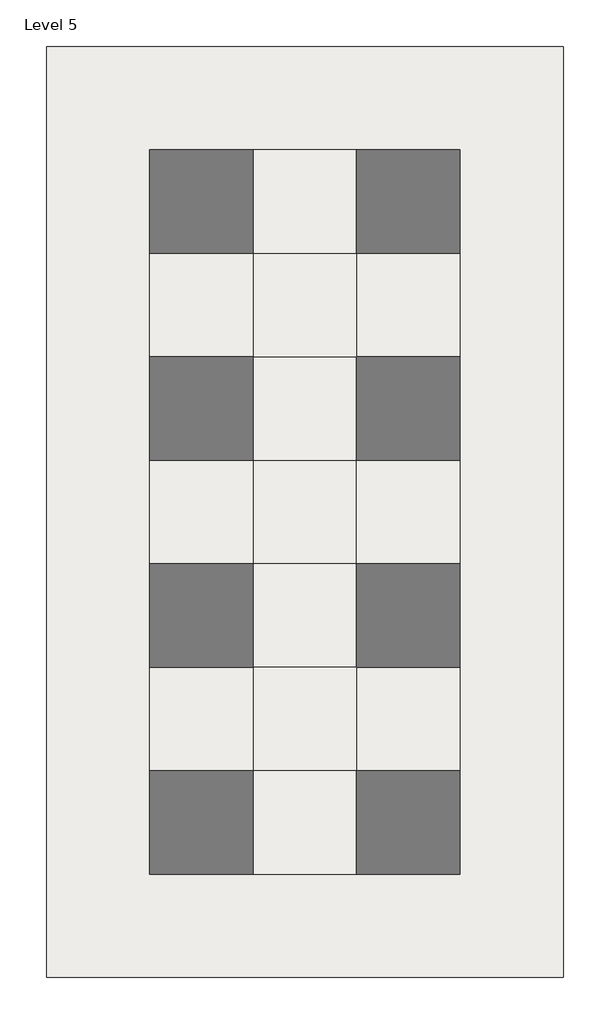
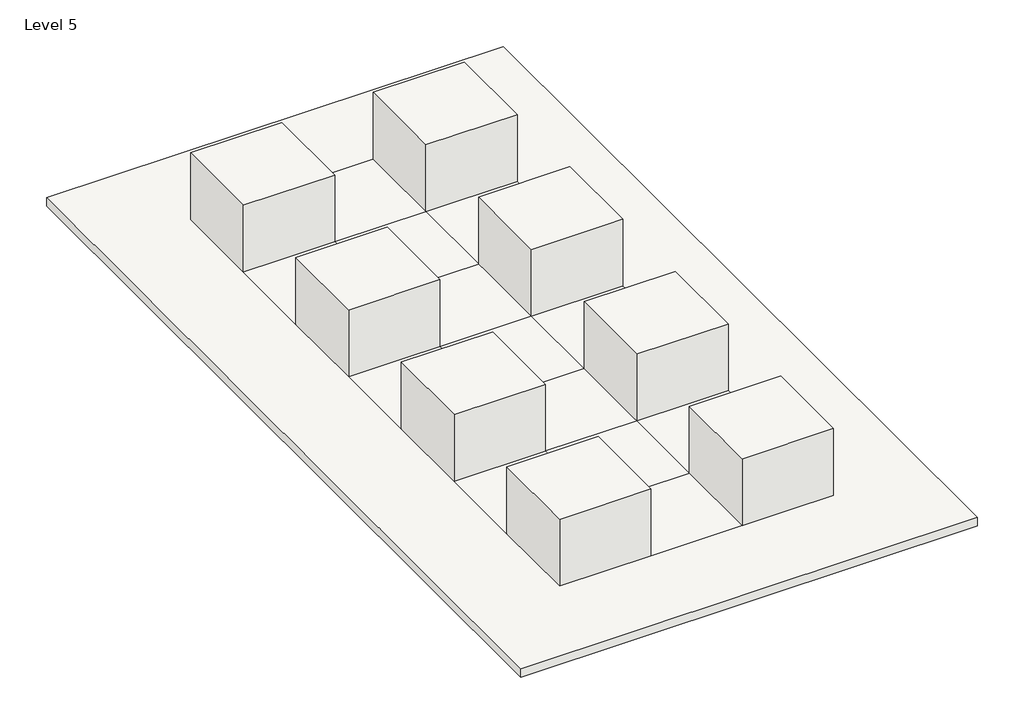
# One storey: 9 roofs.
"""IFC4 building model written with IfcOpenShell, lengths in millimetres."""

from ifc_helpers import new_model, si_unit, origin, place, context, project, spatial, faceted_brep, element, save

model = new_model("IFC4")

# Units and contexts
model_context = context("Model", 3, world=origin())
ifc_project = project(units=[si_unit("LENGTHUNIT", "METRE", prefix="MILLI")], contexts=[model_context])

# Site, building, storey
site = spatial("IfcSite", under=ifc_project)
building = spatial("IfcBuilding", under=site)
storey = spatial("IfcBuildingStorey", under=building, Name="Level 5", Elevation=20000.0)

# Roofs
placement = place(None, origin())
element("IfcRoof", 1, ObjectType="Bauder_RoofCoveringSystem_IntensiveGreenRoofSystem", at=placement, inside=storey, context=model_context, shape_type="Brep", body=[
    faceted_brep([(-674.7340554, 1676.2074539, 20000.0), (1325.2659446, 1676.2074539, 20000.0), (1325.2659446, -323.7925461, 20000.0), (-674.7340554, -323.7925461, 20000.0), (1325.2659446, 1676.2074539, 21749.8), (-674.7340554, 1676.2074539, 21749.8), (-674.7340554, -323.7925461, 21749.8), (1325.2659446, -323.7925461, 21749.8), (1325.2659446, 1676.2074539, 20200.0), (-674.7340554, 1676.2074539, 20200.0), (-674.7340554, -323.7925461, 20200.0), (1325.2659446, -323.7925461, 20200.0)], [[[0, 1, 2, 3]], [[4, 5, 6, 7]], [[5, 4, 8, 1, 0, 9]], [[6, 5, 9, 0, 3, 10]], [[7, 6, 10, 3, 2, 11]], [[4, 7, 11, 2, 1, 8]]]),
])
element("IfcRoof", 2, ObjectType="Bauder_RoofCoveringSystem_IntensiveGreenRoofSystem", at=placement, inside=storey, context=model_context, shape_type="Brep", body=[
    faceted_brep([(3325.2659446, 1676.2074539, 20000.0), (5325.2659446, 1676.2074539, 20000.0), (5325.2659446, -323.7925461, 20000.0), (3325.2659446, -323.7925461, 20000.0), (5325.2659446, 1676.2074539, 21749.8), (3325.2659446, 1676.2074539, 21749.8), (3325.2659446, -323.7925461, 21749.8), (5325.2659446, -323.7925461, 21749.8), (3325.2659446, 1676.2074539, 20200.0), (5325.2659446, 1676.2074539, 20200.0), (3325.2659446, -323.7925461, 20200.0), (5325.2659446, -323.7925461, 20200.0)], [[[0, 1, 2, 3]], [[4, 5, 6, 7]], [[0, 8, 5, 4, 9, 1]], [[3, 10, 6, 5, 8, 0]], [[2, 11, 7, 6, 10, 3]], [[1, 9, 4, 7, 11, 2]]]),
])
element("IfcRoof", 3, ObjectType="Bauder_RoofCoveringSystem_IntensiveGreenRoofSystem", at=placement, inside=storey, context=model_context, shape_type="Brep", body=[
    faceted_brep([(3325.2659446, -2323.7925461, 20000.0), (5325.2659446, -2323.7925461, 20000.0), (5325.2659446, -4323.7925461, 20000.0), (3325.2659446, -4323.7925461, 20000.0), (5325.2659446, -2323.7925461, 21749.8), (3325.2659446, -2323.7925461, 21749.8), (3325.2659446, -4323.7925461, 21749.8), (5325.2659446, -4323.7925461, 21749.8), (3325.2659446, -2323.7925461, 20200.0), (5325.2659446, -2323.7925461, 20200.0), (3325.2659446, -4323.7925461, 20200.0), (5325.2659446, -4323.7925461, 20200.0)], [[[0, 1, 2, 3]], [[4, 5, 6, 7]], [[0, 8, 5, 4, 9, 1]], [[3, 10, 6, 5, 8, 0]], [[2, 11, 7, 6, 10, 3]], [[1, 9, 4, 7, 11, 2]]]),
])
element("IfcRoof", 4, ObjectType="Bauder_RoofCoveringSystem_IntensiveGreenRoofSystem", at=placement, inside=storey, context=model_context, shape_type="Brep", body=[
    faceted_brep([(3325.2659446, -6323.7925461, 20000.0), (5325.2659446, -6323.7925461, 20000.0), (5325.2659446, -8323.7925461, 20000.0), (3325.2659446, -8323.7925461, 20000.0), (5325.2659446, -6323.7925461, 21749.8), (3325.2659446, -6323.7925461, 21749.8), (3325.2659446, -8323.7925461, 21749.8), (5325.2659446, -8323.7925461, 21749.8), (3325.2659446, -6323.7925461, 20200.0), (5325.2659446, -6323.7925461, 20200.0), (3325.2659446, -8323.7925461, 20200.0), (5325.2659446, -8323.7925461, 20200.0)], [[[0, 1, 2, 3]], [[4, 5, 6, 7]], [[0, 8, 5, 4, 9, 1]], [[3, 10, 6, 5, 8, 0]], [[2, 11, 7, 6, 10, 3]], [[1, 9, 4, 7, 11, 2]]]),
])
element("IfcRoof", 5, ObjectType="Bauder_RoofCoveringSystem_IntensiveGreenRoofSystem", at=placement, inside=storey, context=model_context, shape_type="Brep", body=[
    faceted_brep([(3325.2659446, -10323.7925461, 20000.0), (5325.2659446, -10323.7925461, 20000.0), (5325.2659446, -12323.7925461, 20000.0), (3325.2659446, -12323.7925461, 20000.0), (5325.2659446, -10323.7925461, 21749.8), (3325.2659446, -10323.7925461, 21749.8), (3325.2659446, -12323.7925461, 21749.8), (5325.2659446, -12323.7925461, 21749.8), (3325.2659446, -10323.7925461, 20200.0), (5325.2659446, -10323.7925461, 20200.0), (3325.2659446, -12323.7925461, 20200.0), (5325.2659446, -12323.7925461, 20200.0)], [[[0, 1, 2, 3]], [[4, 5, 6, 7]], [[0, 8, 5, 4, 9, 1]], [[3, 10, 6, 5, 8, 0]], [[2, 11, 7, 6, 10, 3]], [[1, 9, 4, 7, 11, 2]]]),
])
element("IfcRoof", 6, ObjectType="Bauder_RoofCoveringSystem_IntensiveGreenRoofSystem", at=placement, inside=storey, context=model_context, shape_type="Brep", body=[
    faceted_brep([(-674.7340554, -10323.7925461, 20000.0), (1325.2659446, -10323.7925461, 20000.0), (1325.2659446, -12323.7925461, 20000.0), (-674.7340554, -12323.7925461, 20000.0), (1325.2659446, -10323.7925461, 21749.8), (-674.7340554, -10323.7925461, 21749.8), (-674.7340554, -12323.7925461, 21749.8), (1325.2659446, -12323.7925461, 21749.8), (-674.7340554, -10323.7925461, 20200.0), (1325.2659446, -10323.7925461, 20200.0), (-674.7340554, -12323.7925461, 20200.0), (1325.2659446, -12323.7925461, 20200.0)], [[[0, 1, 2, 3]], [[4, 5, 6, 7]], [[0, 8, 5, 4, 9, 1]], [[3, 10, 6, 5, 8, 0]], [[2, 11, 7, 6, 10, 3]], [[1, 9, 4, 7, 11, 2]]]),
])
element("IfcRoof", 7, ObjectType="Bauder_RoofCoveringSystem_IntensiveGreenRoofSystem", at=placement, inside=storey, context=model_context, shape_type="Brep", body=[
    faceted_brep([(-674.7340554, -6323.7925461, 20000.0), (1325.2659446, -6323.7925461, 20000.0), (1325.2659446, -8323.7925461, 20000.0), (-674.7340554, -8323.7925461, 20000.0), (1325.2659446, -6323.7925461, 21749.8), (-674.7340554, -6323.7925461, 21749.8), (-674.7340554, -8323.7925461, 21749.8), (1325.2659446, -8323.7925461, 21749.8), (-674.7340554, -6323.7925461, 20200.0), (1325.2659446, -6323.7925461, 20200.0), (-674.7340554, -8323.7925461, 20200.0), (1325.2659446, -8323.7925461, 20200.0)], [[[0, 1, 2, 3]], [[4, 5, 6, 7]], [[0, 8, 5, 4, 9, 1]], [[3, 10, 6, 5, 8, 0]], [[2, 11, 7, 6, 10, 3]], [[1, 9, 4, 7, 11, 2]]]),
])
element("IfcRoof", 8, ObjectType="Bauder_RoofCoveringSystem_IntensiveGreenRoofSystem", at=placement, inside=storey, context=model_context, shape_type="Brep", body=[
    faceted_brep([(-674.7340554, -2323.7925461, 20000.0), (1325.2659446, -2323.7925461, 20000.0), (1325.2659446, -4323.7925461, 20000.0), (-674.7340554, -4323.7925461, 20000.0), (1325.2659446, -2323.7925461, 21749.8), (-674.7340554, -2323.7925461, 21749.8), (-674.7340554, -4323.7925461, 21749.8), (1325.2659446, -4323.7925461, 21749.8), (-674.7340554, -2323.7925461, 20200.0), (1325.2659446, -2323.7925461, 20200.0), (-674.7340554, -4323.7925461, 20200.0), (1325.2659446, -4323.7925461, 20200.0)], [[[0, 1, 2, 3]], [[4, 5, 6, 7]], [[0, 8, 5, 4, 9, 1]], [[3, 10, 6, 5, 8, 0]], [[2, 11, 7, 6, 10, 3]], [[1, 9, 4, 7, 11, 2]]]),
])
element("IfcRoof", 9, ObjectType="Roof_Concrete-200mm", at=placement, inside=storey, context=model_context, shape_type="Brep", body=[
    faceted_brep([(-2674.7340554, -14323.7925461, 20200.0), (-2674.7340554, -14323.7925461, 20000.0), (7325.2659446, -14323.7925461, 20000.0), (7325.2659446, -14323.7925461, 20200.0), (-2674.7340554, 3676.2074539, 20200.0), (-2674.7340554, 3676.2074539, 20000.0), (7325.2659446, 3676.2074539, 20200.0), (7325.2659446, 3676.2074539, 20000.0), (3325.2659446, 1676.2074539, 20200.0), (1325.2659446, 1676.2074539, 20200.0), (1325.2659446, -323.7925461, 20200.0), (3325.2659446, -323.7925461, 20200.0), (1325.2659446, 1676.2074539, 20000.0), (3325.2659446, 1676.2074539, 20000.0), (3325.2659446, -323.7925461, 20000.0), (1325.2659446, -323.7925461, 20000.0), (1325.2659446, -2323.7925461, 20200.0), (-674.7340554, -323.7925461, 20200.0), (-674.7340554, -2323.7925461, 20200.0), (3325.2659446, -2323.7925461, 20200.0), (5325.2659446, -2323.7925461, 20200.0), (5325.2659446, -323.7925461, 20200.0), (-674.7340554, -2323.7925461, 20000.0), (-674.7340554, -323.7925461, 20000.0), (1325.2659446, -2323.7925461, 20000.0), (3325.2659446, -2323.7925461, 20000.0), (5325.2659446, -323.7925461, 20000.0), (5325.2659446, -2323.7925461, 20000.0), (1325.2659446, -4323.7925461, 20200.0), (3325.2659446, -4323.7925461, 20200.0), (3325.2659446, -4323.7925461, 20000.0), (1325.2659446, -4323.7925461, 20000.0), (1325.2659446, -6323.7925461, 20200.0), (-674.7340554, -4323.7925461, 20200.0), (-674.7340554, -6323.7925461, 20200.0), (5325.2659446, -6323.7925461, 20200.0), (5325.2659446, -4323.7925461, 20200.0), (3325.2659446, -6323.7925461, 20200.0), (-674.7340554, -6323.7925461, 20000.0), (-674.7340554, -4323.7925461, 20000.0), (1325.2659446, -6323.7925461, 20000.0), (3325.2659446, -6323.7925461, 20000.0), (5325.2659446, -4323.7925461, 20000.0), (5325.2659446, -6323.7925461, 20000.0), (1325.2659446, -12323.7925461, 20200.0), (3325.2659446, -12323.7925461, 20200.0), (3325.2659446, -10323.7925461, 20200.0), (1325.2659446, -10323.7925461, 20200.0), (3325.2659446, -12323.7925461, 20000.0), (1325.2659446, -12323.7925461, 20000.0), (1325.2659446, -10323.7925461, 20000.0), (3325.2659446, -10323.7925461, 20000.0), (1325.2659446, -8323.7925461, 20200.0), (-674.7340554, -8323.7925461, 20200.0), (-674.7340554, -10323.7925461, 20200.0), (3325.2659446, -8323.7925461, 20200.0), (5325.2659446, -10323.7925461, 20200.0), (5325.2659446, -8323.7925461, 20200.0), (-674.7340554, -10323.7925461, 20000.0), (-674.7340554, -8323.7925461, 20000.0), (1325.2659446, -8323.7925461, 20000.0), (3325.2659446, -8323.7925461, 20000.0), (5325.2659446, -8323.7925461, 20000.0), (5325.2659446, -10323.7925461, 20000.0), (-674.7340554, 1676.2074539, 20000.0), (-674.7340554, 1676.2074539, 20200.0), (5325.2659446, 1676.2074539, 20200.0), (5325.2659446, 1676.2074539, 20000.0), (5325.2659446, -12323.7925461, 20000.0), (5325.2659446, -12323.7925461, 20200.0), (-674.7340554, -12323.7925461, 20000.0), (-674.7340554, -12323.7925461, 20200.0)], [[[0, 1, 2, 3]], [[1, 0, 4, 5]], [[6, 7, 5, 4]], [[3, 2, 7, 6]], [[8, 9, 10, 11]], [[12, 13, 14, 15]], [[16, 10, 17, 18]], [[11, 10, 16, 19]], [[20, 21, 11, 19]], [[22, 23, 15, 24]], [[15, 14, 25, 24]], [[25, 14, 26, 27]], [[19, 16, 28, 29]], [[24, 25, 30, 31]], [[32, 28, 33, 34]], [[35, 36, 29, 37]], [[38, 39, 31, 40]], [[41, 30, 42, 43]], [[44, 45, 46, 47]], [[48, 49, 50, 51]], [[47, 52, 53, 54]], [[47, 46, 55, 52]], [[56, 57, 55, 46]], [[58, 59, 60, 50]], [[51, 50, 60, 61]], [[51, 61, 62, 63]], [[52, 55, 37, 32]], [[29, 28, 32, 37]], [[61, 60, 40, 41]], [[31, 30, 41, 40]], [[9, 12, 15, 10]], [[10, 15, 23, 17]], [[17, 23, 64, 65]], [[12, 9, 65, 64]], [[66, 67, 26, 21]], [[21, 26, 14, 11]], [[11, 14, 13, 8]], [[67, 66, 8, 13]], [[20, 27, 42, 36]], [[36, 42, 30, 29]], [[29, 30, 25, 19]], [[27, 20, 19, 25]], [[16, 24, 31, 28]], [[28, 31, 39, 33]], [[33, 39, 22, 18]], [[24, 16, 18, 22]], [[32, 40, 60, 52]], [[52, 60, 59, 53]], [[53, 59, 38, 34]], [[40, 32, 34, 38]], [[35, 43, 62, 57]], [[57, 62, 61, 55]], [[55, 61, 41, 37]], [[43, 35, 37, 41]], [[56, 63, 68, 69]], [[69, 68, 48, 45]], [[45, 48, 51, 46]], [[63, 56, 46, 51]], [[47, 50, 49, 44]], [[44, 49, 70, 71]], [[71, 70, 58, 54]], [[50, 47, 54, 58]], [[4, 0, 3, 6], [9, 8, 66, 21, 20, 36, 35, 57, 56, 69, 45, 44, 71, 54, 53, 34, 33, 18, 17, 65]], [[7, 2, 1, 5], [13, 12, 64, 23, 22, 39, 38, 59, 58, 70, 49, 48, 68, 63, 62, 43, 42, 27, 26, 67]]]),
])

save(model, "model.ifc")

# Revit data of these elements
# Type "Bauder_RoofCoveringSystem_IntensiveGreenRoofSystem"
#   Keynote = "Q37"
#   Type IFC Predefined Type = "FLAT_ROOF"
#   Export Type to IFC As = "IfcRoofType"
#   Model = "Bauder Intensive Landscaping and Substrate - Intensive Green Roof System"
#   Manufacturer = "Bauder Ltd"
#   Type Comments = "Intensive Green Roof System"
#   URL = "http://www.bauder.co.uk/"
#   Description = "Bauder Intensive GreenRoof system incorporating Intensive Landscaping with Intensive Substrate, Filter Fleece, Mineral Drain, DSE60 Polyethylene Drainage and Protection Layer, FSM 1100 protection mat and PE Foil Polyethylene Separation-Slip Layer"
#   Assembly Code = "B3010"
#   NBSDescription = "Intensive green roof system"
#   NBSReference = "45-40-47/110"
#   BIMObjectName = "Bauder_RoofCoveringSystem_IntensiveGreenRoofSystem"
#   AccessibilityPerformance = "n/a"
#   CodePerformance = "n/a"
#   Color = "n/a"
#   Constituents = "n/a"
#   DurationUnit = "Year"
#   ExpectedLife = "n/a"
#   Features = "This BIM Object must be supported by a project specific specification from Bauder, incorporating system build-up, detail design and performance calculations if a full Bauder system guarantee is required. Please contact your local Bauder Representative or technical@bauder.co.uk"
#   Finish = "n/a"
#   Grade = "n/a"
#   Material = "n/a"
#   ModelReference = "Bauder Intensive Landscaping and Substrate - Intensive Green Roof System"
#   Name = "RoofCoveringSystem_Bauder_IntensiveGreenRoofSystem"
#   ReplacementCost = "n/a"
#   Shape = "n/a"
#   Size = "n/a"
#   SustainabilityPerformance = "Bauder Germany ISO14001: Certificate No.: 70499/03-15 e, Bauder UK ISO14001:Certificate No. 19ACM6595R, EN1271, BREEAM Credits Available"
#   WarrantyDescription = "Guarantee options could include ‘Product’, ‘Product and Workmanship’ and ‘Product, Workmanship and Design’ Guarantees. All guarantees available for this system are subject to the works being carried out in accordance with the Bauder specification and being installed by a Bauder Approved installer. For full details and further information regarding guarantees and alternative systems please contact your local Bauder Representative or technical@bauder.co.uk"
#   WarrantyDurationLabor = "n/a"
#   WarrantyDurationParts = "n/a\r\nn/a"
#   WarrantyDurationUnit = "Year"
#   WarrantyGuarantorLabor = "n/a"
#   WarrantyGuarantorParts = "technical@bauder.co.uk"
#   Certification = "n/a"
#   EdgeRestraints = "Perforated edge trim where required, refer to Bauder Project Specific Specification"
#   MoistureControlDrainageAncillaries = "n/a"
#   MoistureControlDrainageLayer = "Bauder DSE60 60 mm Polyethylene Drainage and Protection Layer with Bauder Mineral Drain Single size stone aggregate infill"
#   MoistureControlFilterMembrane = "Bauder Filter Fleece 1 mm Polypropylene Filter Fleece"
#   MoistureControlMoistureRetentionMat = "n/a"
#   PlantingSystemsAntierosionMat = "Jute Net where exposed, refer to Bauder Project Specific Specification"
#   PlantingSystemsPlantingMedium = "Bauder Intensive Substrate Recycled crushed brick, expanded clay shale and composted pine bark"
#   PlantingSystemsVegetation = "Bauder Intensive Landscaping"
#   PlantingSystemsVegetationBarrier = "20-40 mm Rounded-Washed Stones, refer to Bauder Project Specific Specification"
#   ProjectSpecificationAndDesign = "This BIM Object must be supported by a project specific specification from Bauder, incorporating system build-up, detail design and performance calculations if a full Bauder system warranty is required. Please contact your local Bauder Representative or technical@bauder.co.uk"
#   ProtectionProtectionLayer = "BauderGREEN FSM 1100 Protection Mat"
#   ProtectionRootBarrier = "As per project specific Bauder Specification"
#   ProtectionSeparationLayer = "2 layers of Bauder PE Foil 0.2 mm Polyethylene Separation-Slip Layer"
#   SystemManufacturer = "Bauder Ltd"
#   WarrantyConsiderations = "All guarantees available for this system are subject to the works being carried out in accordance with the Bauder specification and being installed by a Bauder Approved installer. For full details and further information regarding guarantees and alternative systems please contact your local Bauder Representative or technical@bauder.co.uk"
#   Update = "1900-12-31T23:59:59"
#   Documentation = "https://www.bauder.co.uk/technical-centre/technical-literature/system-brochures"
#   DocumentReference = "http://www.bauder.co.uk/"
#   IfcExportAs = "IfcRoofType"
#   IfcExportType = "FLAT_ROOF"
#   MethodOfMesurement = "n/a"
#   Process = "Replacement at service life intervals"
#   FireRating = "n/a"
#   _Author = "AM"
#   _AuthorizedBy = "bimstore"
#   _CreatedBy = "technical@bauder.co.uk"
#   _DistributedBy = "www.bimstore.co"
#   AssetType = "Fixed"
#   ClassificationName = "Uniclass2015"
#   ClassificationValue = "Ss_45_40_47_40"
#   CreatedBy = "technical@bauder.co.uk"
#   CreatedOn = "2023-02-10 T00:00:00"
#   DocumentationCertificates = "n/a"
#   DocumentationInstallationGuide = "https://www.bauder.co.uk/technical-centre"
#   DocumentationLiterature = "https://www.bauder.co.uk/technical-centre"
#   DocumentationMaintenance = "https://www.bauder.co.uk/technical-centre/maintenance-advice"
#   DocumentationTechnical = "https://www.bauder.co.uk/green-roofs/intensive-green-roofs"
#   ManufacturerName = "Bauder Ltd"
#   ModelNumber = "0910_INT-InS-FF-D6-F11-PE"
#   ProductionYear = "2023"
#   ReferencedStandard = "n/a"
#   SpareParts = "n/a"
#   TypeName = "Intensive Green Roof System"
#   NBSNote = "n/a"
#   NBSObjectName = "Bauder - Intensive green roof system"
#   NBSOfficeMasterTag = "n/a"
#   Ballast = "n/a"
#   CarrierMembraneFixing = "n/a"
#   CarrierMembraneType = "n/a"
#   FillToPerimeterUpstands = "n/a"
#   FilterLayer = "n/a"
#   InsulationFixing = "n/a"
#   InsulationType = "n/a"
#   LiquidAppliedWaterproofCoatingReinforcement = "n/a"
#   LiquidAppliedWaterproofCoatingSurfaceTreatment = "n/a"
#   LiquidAppliedWaterproofCoatingType = "n/a"
#   PreparationExistingSubstrates = "n/a"
#   PreparationHorizontalWork = "n/a"
#   PreparationSkirtingsAndVerticalWork = "n/a"
#   ProtectionLayer = "n/a"
#   SystemAccessories = "n/a"
#   WaterproofCoveringFirstLayerAttachment = "n/a"
#   WaterproofCoveringFirstLayerType = "n/a"
#   WaterproofCoveringIntermediateLayerAttachment = "n/a"
#   WaterproofCoveringIntermediateLayerType = "n/a"
#   WaterproofCoveringTopLayerAttachment = "n/a"
#   InsulationAttachment = "n/a"
#   IsolatingLayer = "n/a"
#   CarrierMembraneAttachment = "n/a"
#   LiquidAppliedWaterproofCoatingWearingCourse = "n/a"
#   VapourControlLayer = "n/a"
#   VapourControlLayerAttachment_Bauder = "n/a"
#   WaterproofCoveringJoints = "n/a"
#   WaterproofCoveringType = "n/a"
#   SeparatingLayer = "n/a"
#   WaterproofCoveringAccessories = "Yes"
#   WaterproofCoveringAttachment = "n/a"
#   UpperProtectionLayer = "n/a"
#   LowerProtectionLayer = "n/a"
#   WaterproofCoveringTopLayerType = "n/a"
#   DetailWorkAncillaryItems = "Detail as per project specific Bauder Specification"
#   DetailWorkCoverStrips = "Detail as per project specific Bauder Specification"
#   DetailWorkFlashings = "Detail as per project specific Bauder Specification"
#   DetailWorkSkirtingsAndUpstands = "Detail as per project specific Bauder Specification"
#   DetailWorkWeltedDrips = "Detail as per project specific Bauder Specification"
#   OverlayFixing = "n/a"
#   OverlayType = "n/a"
#   SurfaceProtection = "n/a"
#   VapourControlLayerAttachment = "n/a"
#   VapourControlLayerType = "n/a"
#   Cost = 0
#   NominalHeight = 0 mm
#   NominalLength = 0 mm
#   TotalArea = 0 m²
#   NominalDepth = 0 mm
#   IsExternal = yes
#   _BimSpecGuid = 0
#   _BSBibleVersion = 16
#   _CurrentRevision = 4
#   Layers, outside or top first: 700 mm "Bauder_Landscaping_Intensive" (function 5); 800 mm "Bauder_IntensiveSubstrate_BauderGREEN-SUB-IM-UK" (function 2); 1 mm "Bauder_FilterFleece_BauderGREEN-FV-125-100" (function 2); 40 mm "Bauder_DrainageBoard_BauderGREEN-DSE-40" (function 3); 8 mm "Bauder_ProtectionMat_BauderGREEN-FSM1100" (function 3); 200 mm "Concrete" (function 1); 0.8 mm "Bauder_SeparationAndSlipLayer_BauderGREEN-PE-02" (function 3)
# Type "Roof_Concrete-200mm"
#   Layers, outside or top first: 200 mm "Concrete" (function 1)
# Elements 1, 2, 3, 4, 5, 6, 7, 8 (IfcRoof, "Bauder_RoofCoveringSystem_IntensiveGreenRoofSystem")
#   built-in parameter 1001705 = 71.3576 (stored number, unit not read)
#   built-in parameter 1001710 = 33615
#   Phase Created = New Construction
#   Materials on its faces: "Bauder_SeparationAndSlipLayer_BauderGREEN-PE-02", "Bauder_Landscaping_Intensive"
# Element 9 (IfcRoof, "Roof_Concrete-200mm")
#   built-in parameter 1001710 = 33615
#   Phase Created = New Construction
#   Materials on its faces: "Concrete"
# Materials
#   "Bauder_Landscaping_Intensive": class "Unassigned", colour RGB 62 68 37, transparency 0, Mtrl_Author = "AM", Mtrl_AuthorizedBy = "bimstore", Mtrl_DistributedBy = "www.bimstore.co", Mtrl_AccessibilityPerformance = "n/a", Mtrl_AssetIdentifier = "Please record on commissioning", Mtrl_AssetType = "Fixed", Mtrl_BarCode = "Please record on commissioning", Mtrl_ClassificationName = "Uniclass2015", Mtrl_ClassificationValue = "n/a", Mtrl_CodePerformance = "n/a", Mtrl_Color = "n/a", Mtrl_Constituents = "n/a", Mtrl_CreatedBy = "technical@bauder.co.uk", Mtrl_CreatedOn = "2023-02-10 T00:00:00", Mtrl_DocumentationCertificates = "https://www.bimstore.co/products/intensive-green-roof-system/document/product-certificates", Mtrl_DocumentationInstallationGuide = "https://www.bimstore.co/products/intensive-green-roof-system/document/installation-guide", Mtrl_DocumentationLiterature = "https://www.bimstore.co/products/intensive-green-roof-system/document/product-literature", Mtrl_DocumentationMaintenance = "https://www.bimstore.co/products/intensive-green-roof-system/document/maintenance-information", Mtrl_DocumentationTechnical = "https://www.bimstore.co/products/intensive-green-roof-system/document/technical-data-sheet", Mtrl_DurationUnit = "Year", Mtrl_Features = "n/a", Mtrl_Finish = "n/a", Mtrl_Grade = "n/a", Mtrl_InstallationDate = "Please record on commissioning", Mtrl_ManufacturerName = "Bauder Ltd", Mtrl_Material = "n/a", Mtrl_ModelNumber = "Intensive", Mtrl_ModelReference = "Landscaping", Mtrl_ProductionYear = "2023", Mtrl_ReferencedStandard = "n/a", Mtrl_Shape = "n/a", Mtrl_Size = "n/a", Mtrl_SpareParts = "n/a", Mtrl_TypeName = "Intensive", Mtrl_WarrantyDescription = "n/a", Mtrl_WarrantyDurationUnit = "Year", Mtrl_WarrantyGuarantorLabor = "n/a", Mtrl_WarrantyGuarantorParts = "technical@bauder.co.uk", Mtrl_WarrantyStartDate = "Please record on commissioning", Mtrl_IfcExportAs = "IfcRoofType", Mtrl_IfcExportType = "FLAT_ROOF", Mtrl_BIMObjectName = "Bauder_Landscaping_Intensive", Mtrl_NBSDescription = "n/a", Mtrl_NBSNote = "n/a", Mtrl_NBSObjectName = "n/a", Mtrl_NBSOfficeMasterTag = "n/a", Mtrl_NBSReference = "Q37", Mtrl_Ballast = "n/a", Mtrl_CarrierMembraneAttachment = "n/a", Mtrl_CarrierMembraneFixing = "n/a", Mtrl_CarrierMembraneType = "n/a", Mtrl_Certification = "Comply with GRO Green Roof Code of Practice and FLL Standards", Mtrl_DetailWorkAncillaryItems = "Detail as per project specific Bauder Specification", Mtrl_DetailWorkCoverStrips = "Detail as per project specific Bauder Specification", Mtrl_DetailWorkFlashings = "Detail as per project specific Bauder Specification", Mtrl_DetailWorkSkirtingsAndUpstands = "Detail as per project specific Bauder Specification", Mtrl_DetailWorkWeltedDrips = "Detail as per project specific Bauder Specification", Mtrl_EdgeRestraints = "Detail as per project specific Bauder Specification", Mtrl_FillToPerimeterUpstands = "n/a", Mtrl_FilterLayer = "n/a", Mtrl_InsulationAttachment = "As per project specific Bauder Specification", Mtrl_InsulationFixing = "As per project specific Bauder Specification", Mtrl_InsulationType = "As per project specific Bauder Specification", Mtrl_IsolatingLayer = "n/a", Mtrl_LiquidAppliedWaterproofCoatingReinforcement = "n/a", Mtrl_LiquidAppliedWaterproofCoatingSurfaceTreatment = "As per project specific Bauder Specification", Mtrl_LiquidAppliedWaterproofCoatingType = "As per project specific Bauder Specification", Mtrl_LiquidAppliedWaterproofCoatingWearingCourse = "As per project specific Bauder Specification", Mtrl_LowerProtectionLayer = "n/a", Mtrl_MoistureControlDrainageAncillaries = "n/a", Mtrl_MoistureControlDrainageLayer = "n/a", Mtrl_MoistureControlFilterMembrane = "n/a", Mtrl_MoistureControlMoistureRetentionMat = "n/a", Mtrl_OverlayFixing = "n/a", Mtrl_OverlayType = "n/a", Mtrl_PlantingSystemsAntierosionMat = "n/a", Mtrl_PlantingSystemsPlantingMedium = "As per project specific Bauder Specification", Mtrl_PlantingSystemsVegetation = "As per project specific Bauder Specification", Mtrl_PlantingSystemsVegetationBarrier = "As per project specific Bauder Specification", Mtrl_PreparationExistingSubstrates = "n/a", Mtrl_PreparationHorizontalWork = "n/a", Mtrl_PreparationSkirtingsAndVerticalWork = "n/a", Mtrl_ProjectSpecificationAndDesign = "This BIM Object must be supported by a project specific specification from Bauder, incorporating system build-up, detail design and performance calculations if a full Bauder system warranty is required. Please contact your local Bauder Representative or technical@bauder.co.uk", Mtrl_ProtectionLayer = "n/a", Mtrl_ProtectionProtectionLayer = "n/a", Mtrl_ProtectionRootBarrier = "As per project specific Bauder Specification", Mtrl_ProtectionSeparationLayer = "n/a", Mtrl_SeparatingLayer = "n/a", Mtrl_SurfaceProtection = "n/a", Mtrl_SystemAccessories = "n/a", Mtrl_SystemManufacturer = "Bauder Ltd", Mtrl_Update = "1900-12-31 T23:59:59", Mtrl_UpperProtectionLayer = "n/a", Mtrl_VapourControlLayerAttachment = "As per project specific Bauder Specification", Mtrl_VapourControlLayerAttachment_Bauder = "As per project specific Bauder Specification", Mtrl_VapourControlLayerType = "As per project specific Bauder Specification", Mtrl_WarrantyConsiderations = "All guarantees available for this system are subject to the works being carried out in accordance with the Bauder specification and being installed by a Bauder Approved installer. For full details and further information regarding guarantees and alternative systems please contact your local Bauder Representative or technical@bauder.co.uk", Mtrl_WaterproofCoveringAccessories = "As per project specific Bauder Specification", Mtrl_WaterproofCoveringAttachment = "As per project specific Bauder Specification", Mtrl_WaterproofCoveringFirstLayerAttachment = "As per project specific Bauder Specification", Mtrl_WaterproofCoveringFirstLayerType = "As per project specific Bauder Specification", Mtrl_WaterproofCoveringIntermediateLayerAttachment = "As per project specific Bauder Specification", Mtrl_WaterproofCoveringIntermediateLayerType = "As per project specific Bauder Specification", Mtrl_WaterproofCoveringJoints = "As per project specific Bauder Specification", Mtrl_WaterproofCoveringTopLayerAttachment = "As per project specific Bauder Specification", Mtrl_WaterproofCoveringTopLayerType = "As per project specific Bauder Specification", Mtrl_WaterproofCoveringType = "As per project specific Bauder Specification", Cost = 0, Mtrl_ReplacementCost = 0, Mtrl_NominalDepth = 0 mm, Mtrl_NominalHeight = 0 mm, Mtrl_NominalLength = 0 mm, Mtrl_BimSpecGuid = 0, Mtrl_BSBibleVersion = 17, Mtrl_CurrentRevision = 2, Mtrl_ExpectedLife = 0, Mtrl_SerialNumber = 0, Mtrl_WarrantyDurationLabor = 0, Mtrl_WarrantyDurationParts = 0
#   "Bauder_IntensiveSubstrate_BauderGREEN-SUB-IM-UK": class "Unassigned", colour RGB 255 255 255, transparency 0, Mtrl_Author = "AM", Mtrl_AuthorizedBy = "bimstore", Mtrl_DistributedBy = "www.bimstore.co", Mtrl_AccessibilityPerformance = "n/a", Mtrl_AssetIdentifier = "Please record on commissioning", Mtrl_AssetType = "Fixed", Mtrl_BarCode = "Please record on commissioning", Mtrl_ClassificationName = "Uniclass2015", Mtrl_ClassificationValue = "n/a", Mtrl_CodePerformance = "n/a", Mtrl_Color = "n/a", Mtrl_Constituents = "n/a", Mtrl_CreatedBy = "technical@bauder.co.uk", Mtrl_CreatedOn = "2023-02-10 T00:00:00", Mtrl_DocumentationCertificates = "https://www.bimstore.co/products/intensive-green-roof-system/document/product-certificates", Mtrl_DocumentationInstallationGuide = "https://www.bimstore.co/products/intensive-green-roof-system/document/installation-guide", Mtrl_DocumentationLiterature = "https://www.bimstore.co/products/intensive-green-roof-system/document/product-literature", Mtrl_DocumentationMaintenance = "https://www.bimstore.co/products/intensive-green-roof-system/document/maintenance-information", Mtrl_DocumentationTechnical = "https://www.bimstore.co/products/intensive-green-roof-system/document/technical-data-sheet", Mtrl_DurationUnit = "Year", Mtrl_Features = "n/a", Mtrl_Finish = "n/a", Mtrl_Grade = "n/a", Mtrl_InstallationDate = "Please record on commissioning", Mtrl_ManufacturerName = "Bauder Ltd", Mtrl_Material = "Expanded Clay Aggregate", Mtrl_ModelNumber = "BauderGREEN-SUB-IM-UK", Mtrl_ModelReference = "Intensive Substrate", Mtrl_ProductionYear = "2023", Mtrl_ReferencedStandard = "n/a", Mtrl_Shape = "n/a", Mtrl_Size = "n/a", Mtrl_SpareParts = "n/a", Mtrl_TypeName = "BauderGREEN-SUB-IM-UK", Mtrl_WarrantyDescription = "As part of Bauder system guarantee, per specification", Mtrl_WarrantyDurationUnit = "Year", Mtrl_WarrantyGuarantorLabor = "n/a", Mtrl_WarrantyGuarantorParts = "technical@bauder.co.uk", Mtrl_WarrantyStartDate = "Please record on commissioning", Mtrl_IfcExportAs = "IfcRoofType", Mtrl_IfcExportType = "FLAT_ROOF", Mtrl_BIMObjectName = "Bauder_IntensiveSubstrate_BauderGREEN-SUB-IM-UK", Mtrl_NBSDescription = "n/a", Mtrl_NBSNote = "n/a", Mtrl_NBSObjectName = "n/a", Mtrl_NBSOfficeMasterTag = "n/a", Mtrl_NBSReference = "Q37", Mtrl_Ballast = "n/a", Mtrl_CarrierMembraneAttachment = "n/a", Mtrl_CarrierMembraneFixing = "n/a", Mtrl_CarrierMembraneType = "n/a", Mtrl_Certification = "Comply with GRO Green Roof Code of Practice and FLL Standards", Mtrl_DetailWorkAncillaryItems = "Detail as per project specific Bauder Specification", Mtrl_DetailWorkCoverStrips = "Detail as per project specific Bauder Specification", Mtrl_DetailWorkFlashings = "Detail as per project specific Bauder Specification", Mtrl_DetailWorkSkirtingsAndUpstands = "Detail as per project specific Bauder Specification", Mtrl_DetailWorkWeltedDrips = "Detail as per project specific Bauder Specification", Mtrl_EdgeRestraints = "Detail as per project specific Bauder Specification", Mtrl_FillToPerimeterUpstands = "n/a", Mtrl_FilterLayer = "n/a", Mtrl_InsulationAttachment = "As per project specific Bauder Specification", Mtrl_InsulationFixing = "As per project specific Bauder Specification", Mtrl_InsulationType = "As per project specific Bauder Specification", Mtrl_IsolatingLayer = "n/a", Mtrl_LiquidAppliedWaterproofCoatingReinforcement = "As per project specific Bauder Specification", Mtrl_LiquidAppliedWaterproofCoatingSurfaceTreatment = "As per project specific Bauder Specification", Mtrl_LiquidAppliedWaterproofCoatingType = "As per project specific Bauder Specification", Mtrl_LiquidAppliedWaterproofCoatingWearingCourse = "As per project specific Bauder Specification", Mtrl_LowerProtectionLayer = "n/a", Mtrl_MoistureControlDrainageAncillaries = "n/a", Mtrl_MoistureControlDrainageLayer = "n/a", Mtrl_MoistureControlFilterMembrane = "n/a", Mtrl_MoistureControlMoistureRetentionMat = "n/a", Mtrl_OverlayFixing = "n/a", Mtrl_OverlayType = "n/a", Mtrl_PlantingSystemsAntierosionMat = "n/a", Mtrl_PlantingSystemsPlantingMedium = "As per project specific Bauder Specification", Mtrl_PlantingSystemsVegetation = "As per project specific Bauder Specification", Mtrl_PlantingSystemsVegetationBarrier = "As per project specific Bauder Specification", Mtrl_PreparationExistingSubstrates = "n/a", Mtrl_PreparationHorizontalWork = "n/a", Mtrl_PreparationSkirtingsAndVerticalWork = "n/a", Mtrl_ProjectSpecificationAndDesign = "This BIM Object must be supported by a project specific specification from Bauder, incorporating system build-up, detail design and performance calculations if a full Bauder system warranty is required. Please contact your local Bauder Representative or technical@bauder.co.uk", Mtrl_ProtectionLayer = "n/a", Mtrl_ProtectionProtectionLayer = "n/a", Mtrl_ProtectionRootBarrier = "As per project specific Bauder Specification", Mtrl_ProtectionSeparationLayer = "n/a", Mtrl_SeparatingLayer = "n/a", Mtrl_SurfaceProtection = "n/a", Mtrl_SystemAccessories = "n/a", Mtrl_SystemManufacturer = "Bauder Ltd", Mtrl_Update = "1900-12-31 T23:59:59", Mtrl_UpperProtectionLayer = "n/a", Mtrl_VapourControlLayerAttachment = "As per project specific Bauder Specification", Mtrl_VapourControlLayerAttachment_Bauder = "As per project specific Bauder Specification", Mtrl_VapourControlLayerType = "As per project specific Bauder Specification", Mtrl_WarrantyConsiderations = "All guarantees available for this system are subject to the works being carried out in accordance with the Bauder specification and being installed by a Bauder Approved installer. For full details and further information regarding guarantees and alternative systems please contact your local Bauder Representative or technical@bauder.co.uk", Mtrl_WaterproofCoveringAccessories = "As per project specific Bauder Specification", Mtrl_WaterproofCoveringAttachment = "As per project specific Bauder Specification", Mtrl_WaterproofCoveringFirstLayerAttachment = "As per project specific Bauder Specification", Mtrl_WaterproofCoveringFirstLayerType = "As per project specific Bauder Specification", Mtrl_WaterproofCoveringIntermediateLayerAttachment = "As per project specific Bauder Specification", Mtrl_WaterproofCoveringIntermediateLayerType = "As per project specific Bauder Specification", Mtrl_WaterproofCoveringJoints = "As per project specific Bauder Specification", Mtrl_WaterproofCoveringTopLayerAttachment = "As per project specific Bauder Specification", Mtrl_WaterproofCoveringTopLayerType = "As per project specific Bauder Specification", Mtrl_WaterproofCoveringType = "As per project specific Bauder Specification", Cost = 0, Mtrl_ReplacementCost = 0, Mtrl_NominalDepth = 200 mm, Mtrl_NominalHeight = 0 mm, Mtrl_NominalLength = 0 mm, Mtrl_BimSpecGuid = 0, Mtrl_BSBibleVersion = 17, Mtrl_CurrentRevision = 2, Mtrl_ExpectedLife = 0, Mtrl_SerialNumber = 0, Mtrl_WarrantyDurationLabor = 0, Mtrl_WarrantyDurationParts = 0
#   "Bauder_FilterFleece_BauderGREEN-FV-125-100": class "Unassigned", colour RGB 255 255 255, transparency 0, Mtrl_Author = "AM", Mtrl_AuthorizedBy = "bimstore", Mtrl_DistributedBy = "www.bimstore.co", Mtrl_AccessibilityPerformance = "n/a", Mtrl_AssetIdentifier = "Please record on commissioning", Mtrl_AssetType = "Fixed", Mtrl_BarCode = "Please record on commissioning", Mtrl_ClassificationName = "Uniclass2015", Mtrl_ClassificationValue = "n/a", Mtrl_CodePerformance = "n/a", Mtrl_Color = "n/a", Mtrl_Constituents = "n/a", Mtrl_CreatedBy = "technical@bauder.co.uk", Mtrl_CreatedOn = "2023-02-10 T00:00:00", Mtrl_DocumentationCertificates = "https://www.bimstore.co/products/extensive-green-roof-system-wildflower-blanket/document/product-certificates", Mtrl_DocumentationInstallationGuide = "https://www.bimstore.co/products/extensive-green-roof-system-wildflower-blanket/document/installation-guide", Mtrl_DocumentationLiterature = "https://www.bimstore.co/products/intensive-green-roof-system/document/product-literature", Mtrl_DocumentationMaintenance = "https://www.bimstore.co/products/extensive-green-roof-system-wildflower-blanket/document/maintenance-information", Mtrl_DocumentationTechnical = "https://www.bimstore.co/products/extensive-green-roof-system-wildflower-blanket/document/technical-data-sheet", Mtrl_DurationUnit = "Year", Mtrl_Features = "n/a", Mtrl_Finish = "n/a", Mtrl_Grade = "n/a", Mtrl_InstallationDate = "Please record on commissioning", Mtrl_ManufacturerName = "Bauder Ltd", Mtrl_Material = "Polypropylene Fleece", Mtrl_ModelNumber = "BauderGREEN-FV-125-100", Mtrl_ModelReference = "Filter Fleece", Mtrl_ProductionYear = "2023", Mtrl_ReferencedStandard = "n/a", Mtrl_Shape = "n/a", Mtrl_Size = "n/a", Mtrl_SpareParts = "n/a", Mtrl_TypeName = "BauderGREEN-FV-125-100", Mtrl_WarrantyDescription = "As part of Bauder system guarantee, per specification", Mtrl_WarrantyDurationUnit = "Year", Mtrl_WarrantyGuarantorLabor = "technical@bauder.co.uk", Mtrl_WarrantyGuarantorParts = "technical@bauder.co.uk", Mtrl_WarrantyStartDate = "Please record on commissioning", Mtrl_IfcExportAs = "IfcRoofType", Mtrl_IfcExportType = "FLAT_ROOF", Mtrl_BIMObjectName = "Bauder_FilterFleece_BauderGREEN-FV-125-100", Mtrl_NBSDescription = "n/a", Mtrl_NBSNote = "n/a", Mtrl_NBSObjectName = "n/a", Mtrl_NBSOfficeMasterTag = "n/a", Mtrl_NBSReference = "Q37", Mtrl_Ballast = "n/a", Mtrl_CarrierMembraneAttachment = "n/a", Mtrl_CarrierMembraneFixing = "n/a", Mtrl_CarrierMembraneType = "n/a", Mtrl_Certification = "Comply with GRO Green Roof Code of Practice and FLL Standards", Mtrl_DetailWorkAncillaryItems = "Detail as per project specific Bauder Specification", Mtrl_DetailWorkCoverStrips = "Detail as per project specific Bauder Specification", Mtrl_DetailWorkFlashings = "Detail as per project specific Bauder Specification", Mtrl_DetailWorkSkirtingsAndUpstands = "Detail as per project specific Bauder Specification", Mtrl_DetailWorkWeltedDrips = "Detail as per project specific Bauder Specification", Mtrl_EdgeRestraints = "Detail as per project specific Bauder Specification", Mtrl_FillToPerimeterUpstands = "n/a", Mtrl_FilterLayer = "n/a", Mtrl_InsulationAttachment = "As per project specific Bauder Specification", Mtrl_InsulationFixing = "As per project specific Bauder Specification", Mtrl_InsulationType = "As per project specific Bauder Specification", Mtrl_IsolatingLayer = "n/a", Mtrl_LiquidAppliedWaterproofCoatingReinforcement = "As per project specific Bauder Specification", Mtrl_LiquidAppliedWaterproofCoatingSurfaceTreatment = "As per project specific Bauder Specification", Mtrl_LiquidAppliedWaterproofCoatingType = "As per project specific Bauder Specification", Mtrl_LiquidAppliedWaterproofCoatingWearingCourse = "As per project specific Bauder Specification", Mtrl_LowerProtectionLayer = "n/a", Mtrl_MoistureControlDrainageAncillaries = "n/a", Mtrl_MoistureControlDrainageLayer = "n/a", Mtrl_MoistureControlFilterMembrane = "n/a", Mtrl_MoistureControlMoistureRetentionMat = "n/a", Mtrl_OverlayFixing = "n/a", Mtrl_OverlayType = "n/a", Mtrl_PlantingSystemsAntierosionMat = "n/a", Mtrl_PlantingSystemsPlantingMedium = "As per project specific Bauder Specification", Mtrl_PlantingSystemsVegetation = "As per project specific Bauder Specification", Mtrl_PlantingSystemsVegetationBarrier = "As per project specific Bauder Specification", Mtrl_PreparationExistingSubstrates = "n/a", Mtrl_PreparationHorizontalWork = "n/a", Mtrl_PreparationSkirtingsAndVerticalWork = "n/a", Mtrl_ProjectSpecificationAndDesign = "This BIM Object must be supported by a project specific specification from Bauder, incorporating system build-up, detail design and performance calculations if a full Bauder system warranty is required. Please contact your local Bauder Representative or technical@bauder.co.uk", Mtrl_ProtectionLayer = "n/a", Mtrl_ProtectionProtectionLayer = "n/a", Mtrl_ProtectionRootBarrier = "As per project specific Bauder Specification", Mtrl_ProtectionSeparationLayer = "n/a", Mtrl_SeparatingLayer = "n/a", Mtrl_SurfaceProtection = "n/a", Mtrl_SystemAccessories = "n/a", Mtrl_SystemManufacturer = "Bauder Ltd", Mtrl_Update = "1900-12-31 T23:59:59", Mtrl_UpperProtectionLayer = "n/a", Mtrl_VapourControlLayerAttachment = "As per project specific Bauder Specification", Mtrl_VapourControlLayerAttachment_Bauder = "As per project specific Bauder Specification", Mtrl_VapourControlLayerType = "As per project specific Bauder Specification", Mtrl_WarrantyConsiderations = "All guarantees available for this system are subject to the works being carried out in accordance with the Bauder specification and being installed by a Bauder Approved installer. For full details and further information regarding guarantees and alternative systems please contact your local Bauder Representative or technical@bauder.co.uk", Mtrl_WaterproofCoveringAccessories = "As per project specific Bauder Specification", Mtrl_WaterproofCoveringAttachment = "As per project specific Bauder Specification", Mtrl_WaterproofCoveringFirstLayerAttachment = "As per project specific Bauder Specification", Mtrl_WaterproofCoveringFirstLayerType = "As per project specific Bauder Specification", Mtrl_WaterproofCoveringIntermediateLayerAttachment = "As per project specific Bauder Specification", Mtrl_WaterproofCoveringIntermediateLayerType = "As per project specific Bauder Specification", Mtrl_WaterproofCoveringJoints = "As per project specific Bauder Specification", Mtrl_WaterproofCoveringTopLayerAttachment = "As per project specific Bauder Specification", Mtrl_WaterproofCoveringTopLayerType = "As per project specific Bauder Specification", Mtrl_WaterproofCoveringType = "As per project specific Bauder Specification", Cost = 0, Mtrl_ReplacementCost = 0, Mtrl_NominalDepth = 1 mm, Mtrl_NominalHeight = 0 mm, Mtrl_NominalLength = 0 mm, Mtrl_BimSpecGuid = 0, Mtrl_BSBibleVersion = 17, Mtrl_CurrentRevision = 2, Mtrl_ExpectedLife = 0, Mtrl_SerialNumber = 0, Mtrl_WarrantyDurationLabor = 0, Mtrl_WarrantyDurationParts = 0
#   "Bauder_DrainageBoard_BauderGREEN-DSE-40": class "Unassigned", colour RGB 255 255 255, transparency 0, Mtrl_Author = "AM", Mtrl_AuthorizedBy = "bimstore", Mtrl_DistributedBy = "www.bimstore.co", Mtrl_AccessibilityPerformance = "n/a", Mtrl_AssetIdentifier = "Please record on commissioning", Mtrl_AssetType = "Fixed", Mtrl_BarCode = "Please record on commissioning", Mtrl_ClassificationName = "Uniclass2015", Mtrl_ClassificationValue = "Pr_65_67_78_72", Mtrl_CodePerformance = "n/a", Mtrl_Color = "n/a", Mtrl_Constituents = "n/a", Mtrl_CreatedBy = "technical@bauder.co.uk", Mtrl_CreatedOn = "2023-02-10 T00:00:00", Mtrl_DocumentationCertificates = "https://www.bimstore.co/products/extensive-green-roof-system-wildflower-blanket/document/product-certificates", Mtrl_DocumentationInstallationGuide = "https://www.bimstore.co/products/extensive-green-roof-system-wildflower-blanket/document/installation-guide", Mtrl_DocumentationLiterature = "https://www.bimstore.co/products/extensive-green-roof-system-wildflower-blanket/document/product-literature", Mtrl_DocumentationMaintenance = "https://www.bimstore.co/products/extensive-green-roof-system-wildflower-blanket/document/maintenance-information", Mtrl_DocumentationTechnical = "https://www.bimstore.co/products/extensive-green-roof-system-wildflower-blanket/document/technical-data-sheet", Mtrl_DurationUnit = "Year", Mtrl_Features = "n/a", Mtrl_Finish = "n/a", Mtrl_Grade = "n/a", Mtrl_InstallationDate = "Please record on commissioning", Mtrl_ManufacturerName = "Bauder Ltd", Mtrl_Material = "Recycled High Density Polyethylene", Mtrl_ModelNumber = "BauderGREEN-DSE-40", Mtrl_ModelReference = "Drainage Board", Mtrl_ProductionYear = "2023", Mtrl_ReferencedStandard = "n/a", Mtrl_Shape = "n/a", Mtrl_Size = "n/a", Mtrl_SpareParts = "n/a", Mtrl_TypeName = "BauderGREEN-DSE-40", Mtrl_WarrantyDescription = "As part of Bauder system guarantee, per specification", Mtrl_WarrantyDurationUnit = "Year", Mtrl_WarrantyGuarantorLabor = "technical@bauder.co.uk", Mtrl_WarrantyGuarantorParts = "technical@bauder.co.uk", Mtrl_WarrantyStartDate = "Please record on commissioning", Mtrl_IfcExportAs = "IfcRoofType", Mtrl_IfcExportType = "FLAT_ROOF", Mtrl_BIMObjectName = "Bauder_DrainageBoard_BauderGREEN-DSE-40", Mtrl_NBSDescription = "n/a", Mtrl_NBSNote = "n/a", Mtrl_NBSObjectName = "n/a", Mtrl_NBSOfficeMasterTag = "n/a", Mtrl_NBSReference = "Q37", Mtrl_Ballast = "n/a", Mtrl_CarrierMembraneAttachment = "n/a", Mtrl_CarrierMembraneFixing = "n/a", Mtrl_CarrierMembraneType = "n/a", Mtrl_Certification = "Comply with GRO Green Roof Code of Practice and FLL Standards", Mtrl_DetailWorkAncillaryItems = "Detail as per project specific Bauder Specification", Mtrl_DetailWorkCoverStrips = "Detail as per project specific Bauder Specification", Mtrl_DetailWorkFlashings = "Detail as per project specific Bauder Specification", Mtrl_DetailWorkSkirtingsAndUpstands = "Detail as per project specific Bauder Specification", Mtrl_DetailWorkWeltedDrips = "Detail as per project specific Bauder Specification", Mtrl_EdgeRestraints = "Detail as per project specific Bauder Specification", Mtrl_FillToPerimeterUpstands = "n/a", Mtrl_FilterLayer = "n/a", Mtrl_InsulationAttachment = "As per project specific Bauder Specification", Mtrl_InsulationFixing = "As per project specific Bauder Specification", Mtrl_InsulationType = "As per project specific Bauder Specification", Mtrl_IsolatingLayer = "n/a", Mtrl_LiquidAppliedWaterproofCoatingReinforcement = "As per project specific Bauder Specification", Mtrl_LiquidAppliedWaterproofCoatingSurfaceTreatment = "As per project specific Bauder Specification", Mtrl_LiquidAppliedWaterproofCoatingType = "As per project specific Bauder Specification", Mtrl_LiquidAppliedWaterproofCoatingWearingCourse = "As per project specific Bauder Specification", Mtrl_LowerProtectionLayer = "n/a", Mtrl_MoistureControlDrainageAncillaries = "n/a", Mtrl_MoistureControlDrainageLayer = "n/a", Mtrl_MoistureControlFilterMembrane = "n/a", Mtrl_MoistureControlMoistureRetentionMat = "n/a", Mtrl_OverlayFixing = "n/a", Mtrl_OverlayType = "n/a", Mtrl_PlantingSystemsAntierosionMat = "n/a", Mtrl_PlantingSystemsPlantingMedium = "As per project specific Bauder Specification", Mtrl_PlantingSystemsVegetation = "As per project specific Bauder Specification", Mtrl_PlantingSystemsVegetationBarrier = "As per project specific Bauder Specification", Mtrl_PreparationExistingSubstrates = "n/a", Mtrl_PreparationHorizontalWork = "n/a", Mtrl_PreparationSkirtingsAndVerticalWork = "n/a", Mtrl_ProjectSpecificationAndDesign = "This BIM Object must be supported by a project specific specification from Bauder, incorporating system build-up, detail design and performance calculations if a full Bauder system warranty is required. Please contact your local Bauder Representative or technical@bauder.co.uk", Mtrl_ProtectionLayer = "n/a", Mtrl_ProtectionProtectionLayer = "n/a", Mtrl_ProtectionRootBarrier = "As per project specific Bauder Specification", Mtrl_ProtectionSeparationLayer = "n/a", Mtrl_SeparatingLayer = "n/a", Mtrl_SurfaceProtection = "n/a", Mtrl_SystemAccessories = "n/a", Mtrl_SystemManufacturer = "Bauder Ltd", Mtrl_Update = "1900-12-31 T23:59:59", Mtrl_UpperProtectionLayer = "n/a", Mtrl_VapourControlLayerAttachment = "As per project specific Bauder Specification", Mtrl_VapourControlLayerAttachment_Bauder = "As per project specific Bauder Specification", Mtrl_VapourControlLayerType = "As per project specific Bauder Specification", Mtrl_WarrantyConsiderations = "All guarantees available for this system are subject to the works being carried out in accordance with the Bauder specification and being installed by a Bauder Approved installer. For full details and further information regarding guarantees and alternative systems please contact your local Bauder Representative or technical@bauder.co.uk", Mtrl_WaterproofCoveringAccessories = "As per project specific Bauder Specification", Mtrl_WaterproofCoveringAttachment = "As per project specific Bauder Specification", Mtrl_WaterproofCoveringFirstLayerAttachment = "As per project specific Bauder Specification", Mtrl_WaterproofCoveringFirstLayerType = "As per project specific Bauder Specification", Mtrl_WaterproofCoveringIntermediateLayerAttachment = "As per project specific Bauder Specification", Mtrl_WaterproofCoveringIntermediateLayerType = "As per project specific Bauder Specification", Mtrl_WaterproofCoveringJoints = "As per project specific Bauder Specification", Mtrl_WaterproofCoveringTopLayerAttachment = "As per project specific Bauder Specification", Mtrl_WaterproofCoveringTopLayerType = "As per project specific Bauder Specification", Mtrl_WaterproofCoveringType = "As per project specific Bauder Specification", Cost = 0, Mtrl_ReplacementCost = 0, Mtrl_NominalDepth = 40 mm, Mtrl_NominalHeight = 0 mm, Mtrl_NominalLength = 0 mm, Mtrl_BimSpecGuid = 0, Mtrl_BSBibleVersion = 17, Mtrl_CurrentRevision = 2, Mtrl_ExpectedLife = 0, Mtrl_SerialNumber = 0, Mtrl_WarrantyDurationLabor = 0, Mtrl_WarrantyDurationParts = 0
#   "Bauder_ProtectionMat_BauderGREEN-FSM1100": class "Unassigned", colour RGB 255 255 255, transparency 0, Mtrl_Author = "AM", Mtrl_AuthorizedBy = "bimstore", Mtrl_DistributedBy = "www.bimstore.co", Mtrl_AccessibilityPerformance = "n/a", Mtrl_AssetIdentifier = "Please record on commissioning", Mtrl_AssetType = "Fixed", Mtrl_BarCode = "Please record on commissioning", Mtrl_ClassificationName = "Uniclass2015", Mtrl_ClassificationValue = "Pr_20_96_71_64", Mtrl_CodePerformance = "n/a", Mtrl_Color = "n/a", Mtrl_Constituents = "n/a", Mtrl_CreatedBy = "technical@bauder.co.uk", Mtrl_CreatedOn = "2023-05-02 T00:00:00", Mtrl_DocumentationCertificates = "https://www.bimstore.co/products/intensive-green-roof-system/document/product-certificates", Mtrl_DocumentationInstallationGuide = "https://www.bimstore.co/products/intensive-green-roof-system/document/installation-guide", Mtrl_DocumentationLiterature = "https://www.bimstore.co/products/intensive-green-roof-system/document/product-literature", Mtrl_DocumentationMaintenance = "https://www.bimstore.co/products/intensive-green-roof-system/document/maintenance-information", Mtrl_DocumentationTechnical = "https://www.bimstore.co/products/intensive-green-roof-system/document/technical-data-sheet", Mtrl_DurationUnit = "Year", Mtrl_Features = "n/a", Mtrl_Finish = "n/a", Mtrl_Grade = "n/a", Mtrl_InstallationDate = "Please record on commissioning", Mtrl_ManufacturerName = "Bauder Ltd", Mtrl_Material = "Polyester and Polypropylene Fibre", Mtrl_ModelNumber = "BauderGREEN FSM1100", Mtrl_ModelReference = "Protection Mat", Mtrl_ProductionYear = "2023", Mtrl_ReferencedStandard = "n/a", Mtrl_Shape = "n/a", Mtrl_Size = "n/a", Mtrl_SpareParts = "n/a", Mtrl_TypeName = "BauderGREEN FSM1100", Mtrl_WarrantyDescription = "As part of Bauder system guarantee, per specification", Mtrl_WarrantyDurationUnit = "Year", Mtrl_WarrantyGuarantorLabor = "n/a", Mtrl_WarrantyGuarantorParts = "technical@bauder.co.uk", Mtrl_WarrantyStartDate = "Please record on commissioning", Mtrl_IfcExportAs = "IfcRoofType", Mtrl_IfcExportType = "FLAT_ROOF", Mtrl_BIMObjectName = "Bauder_ProtectionMat_BauderGREEN-FSM1100", Mtrl_NBSDescription = "n/a", Mtrl_NBSNote = "n/a", Mtrl_NBSObjectName = "n/a", Mtrl_NBSOfficeMasterTag = "n/a", Mtrl_NBSReference = "Q37", Mtrl_Ballast = "n/a", Mtrl_CarrierMembraneAttachment = "n/a", Mtrl_CarrierMembraneFixing = "n/a", Mtrl_CarrierMembraneType = "n/a", Mtrl_Certification = "Comply with GRO Green Roof Code of Practice and FLL Standards", Mtrl_DetailWorkAncillaryItems = "Detail as per project specific Bauder Specification", Mtrl_DetailWorkCoverStrips = "Detail as per project specific Bauder Specification", Mtrl_DetailWorkFlashings = "Detail as per project specific Bauder Specification", Mtrl_DetailWorkSkirtingsAndUpstands = "Detail as per project specific Bauder Specification", Mtrl_DetailWorkWeltedDrips = "Detail as per project specific Bauder Specification", Mtrl_EdgeRestraints = "Detail as per project specific Bauder Specification", Mtrl_FillToPerimeterUpstands = "n/a", Mtrl_FilterLayer = "n/a", Mtrl_InsulationAttachment = "As per project specific Bauder Specification", Mtrl_InsulationFixing = "As per project specific Bauder Specification", Mtrl_InsulationType = "As per project specific Bauder Specification", Mtrl_IsolatingLayer = "n/a", Mtrl_LiquidAppliedWaterproofCoatingReinforcement = "As per project specific Bauder Specification", Mtrl_LiquidAppliedWaterproofCoatingSurfaceTreatment = "As per project specific Bauder Specification", Mtrl_LiquidAppliedWaterproofCoatingType = "As per project specific Bauder Specification", Mtrl_LiquidAppliedWaterproofCoatingWearingCourse = "As per project specific Bauder Specification", Mtrl_LowerProtectionLayer = "n/a", Mtrl_MoistureControlDrainageAncillaries = "n/a", Mtrl_MoistureControlDrainageLayer = "n/a", Mtrl_MoistureControlFilterMembrane = "n/a", Mtrl_MoistureControlMoistureRetentionMat = "n/a", Mtrl_OverlayFixing = "n/a", Mtrl_OverlayType = "n/a", Mtrl_PlantingSystemsAntierosionMat = "n/a", Mtrl_PlantingSystemsPlantingMedium = "As per project specific Bauder Specification", Mtrl_PlantingSystemsVegetation = "As per project specific Bauder Specification", Mtrl_PlantingSystemsVegetationBarrier = "As per project specific Bauder Specification", Mtrl_PreparationExistingSubstrates = "n/a", Mtrl_PreparationHorizontalWork = "n/a", Mtrl_PreparationSkirtingsAndVerticalWork = "n/a", Mtrl_ProjectSpecificationAndDesign = "This BIM Object must be supported by a project specific specification from Bauder, incorporating system build-up, detail design and performance calculations if a full Bauder system warranty is required. Please contact your local Bauder Representative or technical@bauder.co.uk", Mtrl_ProtectionLayer = "n/a", Mtrl_ProtectionProtectionLayer = "n/a", Mtrl_ProtectionRootBarrier = "As per project specific Bauder Specification", Mtrl_ProtectionSeparationLayer = "n/a", Mtrl_SeparatingLayer = "n/a", Mtrl_SurfaceProtection = "n/a", Mtrl_SystemAccessories = "n/a", Mtrl_SystemManufacturer = "Bauder Ltd", Mtrl_Update = "1900-12-31 T23:59:59", Mtrl_UpperProtectionLayer = "n/a", Mtrl_VapourControlLayerAttachment = "As per project specific Bauder Specification", Mtrl_VapourControlLayerAttachment_Bauder = "As per project specific Bauder Specification", Mtrl_VapourControlLayerType = "As per project specific Bauder Specification", Mtrl_WarrantyConsiderations = "All guarantees available for this system are subject to the works being carried out in accordance with the Bauder specification and being installed by a Bauder Approved installer. For full details and further information regarding guarantees and alternative systems please contact your local Bauder Representative or technical@bauder.co.uk", Mtrl_WaterproofCoveringAccessories = "As per project specific Bauder Specification", Mtrl_WaterproofCoveringAttachment = "As per project specific Bauder Specification", Mtrl_WaterproofCoveringFirstLayerAttachment = "As per project specific Bauder Specification", Mtrl_WaterproofCoveringFirstLayerType = "As per project specific Bauder Specification", Mtrl_WaterproofCoveringIntermediateLayerAttachment = "As per project specific Bauder Specification", Mtrl_WaterproofCoveringIntermediateLayerType = "As per project specific Bauder Specification", Mtrl_WaterproofCoveringJoints = "As per project specific Bauder Specification", Mtrl_WaterproofCoveringTopLayerAttachment = "As per project specific Bauder Specification", Mtrl_WaterproofCoveringTopLayerType = "As per project specific Bauder Specification", Mtrl_WaterproofCoveringType = "As per project specific Bauder Specification", Cost = 0, Mtrl_ReplacementCost = 0, Mtrl_NominalDepth = 8 mm, Mtrl_NominalHeight = 0 mm, Mtrl_NominalLength = 0 mm, Mtrl_BimSpecGuid = 0, Mtrl_BSBibleVersion = 17, Mtrl_CurrentRevision = 2, Mtrl_ExpectedLife = 0, Mtrl_SerialNumber = 0, Mtrl_WarrantyDurationLabor = 0, Mtrl_WarrantyDurationParts = 0
#   "Concrete": class "Concrete", colour RGB 120 120 120, transparency 0, Description = "Portland Cement Concrete", Cost = 0
